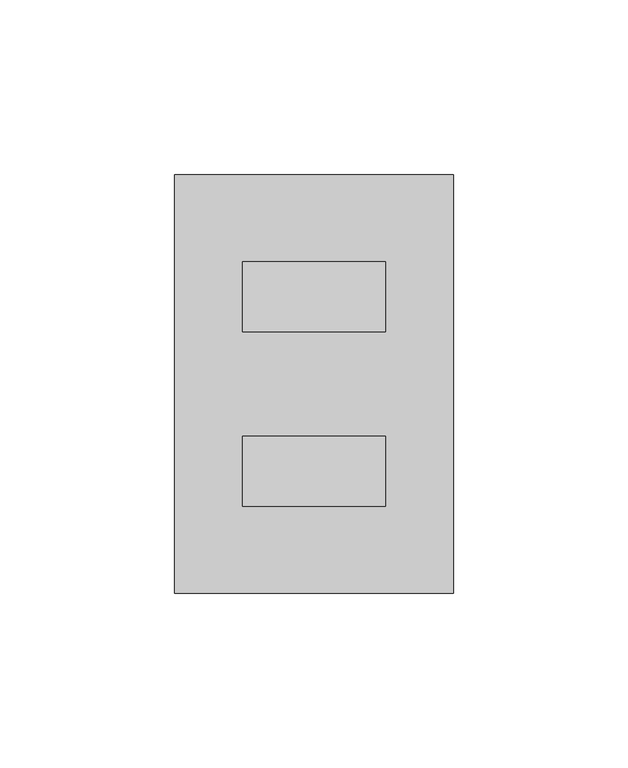
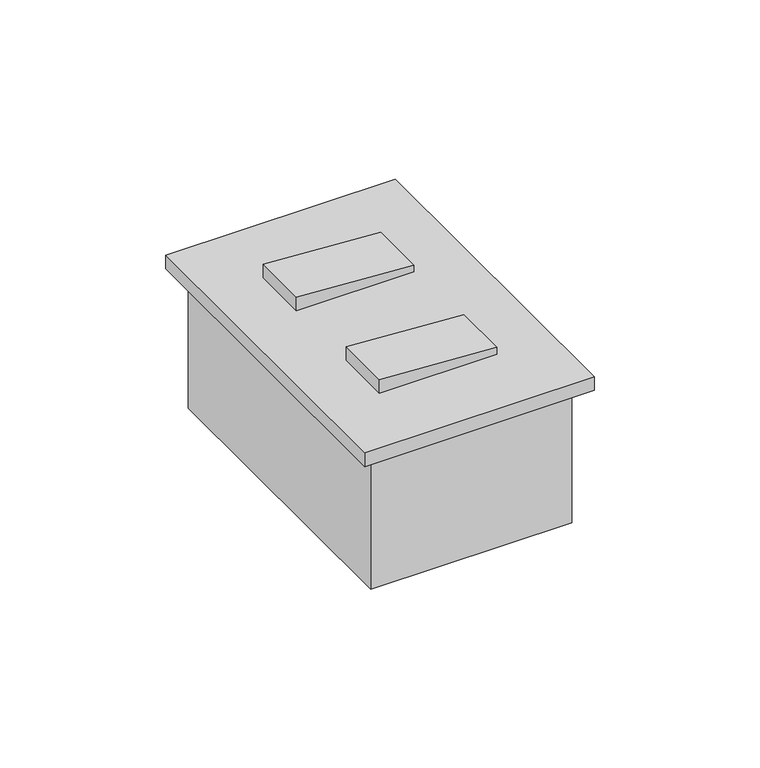
"""IFC4 building model written with IfcOpenShell, lengths in millimetres: proxy geometry, CAIXA VERTICE V7 : Interruptor 2s."""

from ifc_helpers import new_model, si_unit, frame, origin, origin_with_axes, place, context, project, spatial, polyline, outline, extrude, faceted_brep, source, transform, mapped, element, save


def electrical_fixtures_c6f7cd8e(model_context):
    return source(origin(), model_context, "Body", "SolidModel", [
        extrude(outline(polyline([(5.0, 20.5), (7.5, 20.5), (10.0, -20.5), (5.0, -20.5), (5.0, 20.5)])), frame((0.0, 1065.0, 0.0), z_axis=(0.0, 1.0, 0.0), x_axis=(0.0, 0.0, 1.0)), (0.0, 0.0, 1.0), 20.0),
        extrude(outline(polyline([(5.0, 20.5), (7.5, 20.5), (10.0, -20.5), (5.0, -20.5), (5.0, 20.5)])), frame((0.0, 1115.0, 0.0), z_axis=(0.0, 1.0, 0.0), x_axis=(0.0, 0.0, 1.0)), (0.0, 0.0, 1.0), 20.0),
        faceted_brep([(35.0, 1155.0, 0.0), (-35.0, 1155.0, 0.0), (-35.0, 1045.0, 0.0), (35.0, 1045.0, 0.0), (33.0, 1153.0, 0.0), (33.0, 1047.0, 0.0), (-33.0, 1047.0, 0.0), (-33.0, 1153.0, 0.0), (33.0, 1047.0, -48.0), (33.0, 1153.0, -48.0), (-33.0, 1153.0, -48.0), (-33.0, 1047.0, -48.0), (35.0, 1155.0, -50.0), (35.0, 1045.0, -50.0), (-35.0, 1045.0, -50.0), (-35.0, 1155.0, -50.0)], [[[0, 1, 2, 3], [4, 5, 6, 7]], [[8, 9, 10, 11]], [[12, 13, 14, 15]], [[12, 15, 1, 0]], [[1, 15, 14, 2]], [[2, 14, 13, 3]], [[3, 13, 12, 0]], [[5, 4, 9, 8]], [[6, 5, 8, 11]], [[7, 6, 11, 10]], [[4, 7, 10, 9]]]),
        extrude(outline(polyline([(40.0, 1160.0), (40.0, 1040.0), (-40.0, 1040.0), (-40.0, 1160.0), (40.0, 1160.0)])), origin_with_axes(), (0.0, 0.0, 1.0), 5.0),
    ])


if __name__ == "__main__":
    model = new_model("IFC4")
    model_context = context("Model", 3, world=origin())
    ifc_project = project(units=[si_unit("LENGTHUNIT", "METRE", prefix="MILLI")], contexts=[model_context])
    site = spatial("IfcSite", under=ifc_project)
    building = spatial("IfcBuilding", under=site)
    placement = place(None, origin())
    electrical_fixtures_shape = electrical_fixtures_c6f7cd8e(model_context)
    element("IfcBuildingElementProxy", 1, Name="CAIXA VERTICE V7 : Interruptor 2s", ObjectType="CAIXA VERTICE V7 : Interruptor 2s", at=placement, inside=building, context=model_context, shape_type="MappedRepresentation", body=[
        mapped(electrical_fixtures_shape, transform((0.0, 0.0, 0.0), x_axis=(1.0, 0.0, 0.0), y_axis=(0.0, 1.0, 0.0), z_axis=(0.0, 0.0, 1.0))),
    ])
    save(model, "model.ifc")

# Revit data of these elements
# Type "CAIXA VERTICE V7 : Interruptor 2s"
#   URL = "www.facebook.com/verticetreinamentos"
#   SEÇÃO [instance default] = ""
#   Rotação [instance default] = 0.00°
#   LARGURA DA TAMPA = 0.08 m
#   BORDA = 0.01 m
#   ALTURA DE INSTALAÇÃO [instance default] = 1.10 m
#   Distância Anotação [instance default] = 0.0015 m
#   ALTURA DA TAMPA = 0.12 m
#   Vertical [instance default] = yes
#   VER SEÇÃO [instance default] = yes
#   SHADE ESQ [instance default] = no
#   SHADE DIR [instance default] = yes
#   HORIZONTAL [instance default] = no
#   ANDAR COM A LEGENDA [instance default] = 0
#   Material Tampa [instance default] = Plástico, branco opaco
#   Caixa = element 1798510
#   Anotação = element 1798523
#   Default Elevation = 0
# Element 1 (IfcBuildingElementProxy, "CAIXA VERTICE V7 : Interruptor 2s")
#   SEÇÃO = "2"
#   Distância Anotação = 0.0055 m
#   ANDAR COM A LEGENDA = 2
#   Materials on its faces: "Plástico, branco opaco"
# Materials
#   "Plástico, branco opaco": class "Plástico", colour RGB 120 120 120, transparency 0, Description = "Plastic, generic, opaque white", Cost = 0
